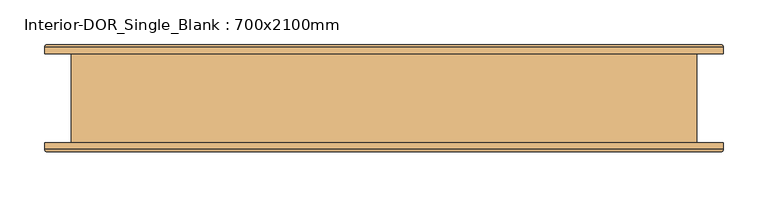
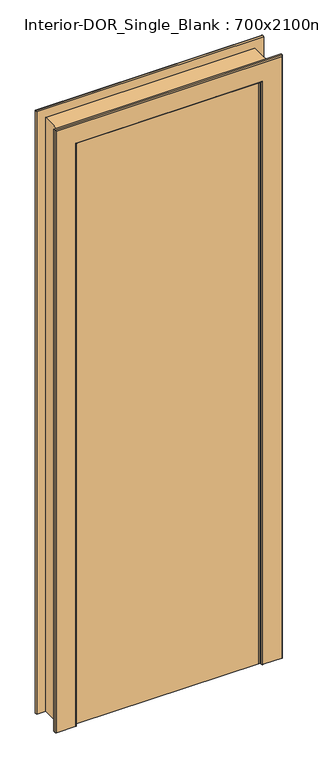
"""IFC4 building model written with IfcOpenShell, lengths in millimetres: door geometry, Interior-DOR_Single_Blank : 700x2100mm."""

import ifcopenshell
import ifcopenshell.guid

model = None  # the IFC model being written
_history = None  # IfcOwnerHistory: only IFC2X3 demands one
_inside = {}  # id of a spatial element -> (the spatial element, [elements in it])
_under = {}  # id of a project, library or spatial element -> (it, [spatial elements below it])
_declared = {}  # id of a project -> (the project, [libraries it declares])
_typed = {}  # id of a type object -> (the type object, [elements of that type])
_made_of = {}  # id of a material, layer set ... -> (it, [elements and type objects made of it])


def new_model(schema):
    """Start an empty IFC model of exactly this schema.

    Asked for "IFC4X3", IfcOpenShell would pick the latest addendum, in which some entities
    have other attributes; the version numbers below select the first issue.
    IFC2X3 requires an IfcOwnerHistory on every rooted entity: one is made here for all.
    """
    global model, _history
    if schema == "IFC4X3":
        model = ifcopenshell.file(schema_version=(4, 3, 0, 0))
    else:
        model = ifcopenshell.file(schema=schema)
    _inside.clear()
    _under.clear()
    _declared.clear()
    _typed.clear()
    _made_of.clear()
    _history = None
    if model.schema == "IFC2X3":
        org = make("IfcOrganization", Name="unknown")
        user = make(
            "IfcPersonAndOrganization",
            ThePerson=make("IfcPerson", FamilyName="unknown"),
            TheOrganization=org,
        )
        app = make(
            "IfcApplication",
            ApplicationDeveloper=org,
            Version="unknown",
            ApplicationFullName="unknown",
            ApplicationIdentifier="unknown",
        )
        _history = make(
            "IfcOwnerHistory",
            OwningUser=user,
            OwningApplication=app,
            ChangeAction="ADDED",
            CreationDate=0,
        )
    return model


def make(cls, **values):
    """One entity of the class cls with the attributes given. An attribute that is None is left unset."""
    return model.create_entity(
        cls, **{name: value for name, value in values.items() if value is not None}
    )


def rooted(cls, **values):
    """An entity with a GlobalId (a new one), such as an element, a storey or a relation."""
    return make(cls, GlobalId=ifcopenshell.guid.new(), OwnerHistory=_history, **values)


def si_unit(unit_type, name, prefix=None):
    """IfcSIUnit, for example si_unit("LENGTHUNIT", "METRE", prefix="MILLI")."""
    return make("IfcSIUnit", UnitType=unit_type, Prefix=prefix, Name=name)


def assignment(units):
    """IfcUnitAssignment: the units of a project."""
    return None if units is None else make("IfcUnitAssignment", Units=units)


def point(xyz):
    """IfcCartesianPoint."""
    return None if xyz is None else make("IfcCartesianPoint", Coordinates=xyz)


def direction(xyz):
    """IfcDirection."""
    return None if xyz is None else make("IfcDirection", DirectionRatios=xyz)


def frame(location, z_axis=None, x_axis=None):
    """IfcAxis2Placement3D, a coordinate frame: its origin and axes. An axis left out is left unset."""
    return make(
        "IfcAxis2Placement3D",
        Location=point(location),
        Axis=direction(z_axis),
        RefDirection=direction(x_axis),
    )


def origin():
    """The frame at (0, 0, 0) with its axes left unset."""
    return frame((0.0, 0.0, 0.0))


def origin_with_axes():
    """The frame at (0, 0, 0) with the z axis (0, 0, 1) and the x axis (1, 0, 0) written out."""
    return frame((0.0, 0.0, 0.0), z_axis=(0.0, 0.0, 1.0), x_axis=(1.0, 0.0, 0.0))


def place(relative_to, where):
    """IfcLocalPlacement: puts the frame where relative to a parent placement (None: the world)."""
    return make(
        "IfcLocalPlacement", PlacementRelTo=relative_to, RelativePlacement=where
    )


def context(
    kind, dimensions, precision=None, world=None, true_north=None, identifier=None
):
    """IfcGeometricRepresentationContext, for example the 3D "Model" context."""
    return make(
        "IfcGeometricRepresentationContext",
        ContextIdentifier=identifier,
        ContextType=kind,
        CoordinateSpaceDimension=dimensions,
        Precision=precision,
        WorldCoordinateSystem=world,
        TrueNorth=true_north,
    )


def project(units=None, contexts=None):
    """IfcProject with its units and contexts."""
    return rooted(
        "IfcProject",
        Name="project",
        RepresentationContexts=contexts,
        UnitsInContext=assignment(units),
    )


def spatial(cls, under=None, at=None, **own):
    """A site, building, storey or space (cls), placed at a placement, below another one or the project."""
    s = rooted(cls, ObjectPlacement=at, **own)
    if under is not None:
        _under.setdefault(under.id(), (under, []))[1].append(s)
    return s


def polyline(points):
    """IfcPolyline through the points."""
    return make("IfcPolyline", Points=[point(p) for p in points])


def circle_curve(where, radius):
    """IfcCircle in the frame where."""
    return make("IfcCircle", Position=where, Radius=radius)


def ellipse_curve(where, semi_axis1, semi_axis2):
    """IfcEllipse in the frame where."""
    return make(
        "IfcEllipse", Position=where, SemiAxis1=semi_axis1, SemiAxis2=semi_axis2
    )


def outline(outer, holes=None, kind="AREA"):
    """IfcArbitraryClosedProfileDef: a profile drawn as a closed curve; with holes, ...WithVoids."""
    if holes is None:
        return make("IfcArbitraryClosedProfileDef", ProfileType=kind, OuterCurve=outer)
    return make(
        "IfcArbitraryProfileDefWithVoids",
        ProfileType=kind,
        OuterCurve=outer,
        InnerCurves=holes,
    )


def extrude(swept, where, along, depth):
    """IfcExtrudedAreaSolid: the profile swept, set in the frame where, extruded along a direction by depth."""
    return make(
        "IfcExtrudedAreaSolid",
        SweptArea=swept,
        Position=where,
        ExtrudedDirection=direction(along),
        Depth=depth,
    )


def faces_of(points, faces, orient=None, outer=None):
    """IfcFace entities. A face is a list of loops; a loop is a list of indices into points, from 0.

    orient and outer hold one flag for each loop. By default every Orientation is true, the
    first loop of a face is its IfcFaceOuterBound and the others are IfcFaceBound.
    """
    made = []
    for i, loops in enumerate(faces):
        bounds = []
        for j, loop in enumerate(loops):
            is_outer = j == 0 if outer is None else outer[i][j]
            bounds.append(
                make(
                    "IfcFaceOuterBound" if is_outer else "IfcFaceBound",
                    Bound=make("IfcPolyLoop", Polygon=[points[k] for k in loop]),
                    Orientation=True if orient is None else orient[i][j],
                )
            )
        made.append(make("IfcFace", Bounds=bounds))
    return made


def faceted_brep(points, faces, orient=None, outer=None, voids=None):
    """IfcFacetedBrep: a solid bounded by flat faces; with voids (closed shells), ...WithVoids."""
    shared = [point(p) for p in points]
    hull = make("IfcClosedShell", CfsFaces=faces_of(shared, faces, orient, outer))
    if voids is None:
        return make("IfcFacetedBrep", Outer=hull)
    return make(
        "IfcFacetedBrepWithVoids",
        Outer=hull,
        Voids=[
            make(cls, CfsFaces=faces_of(shared, fs, o, b)) for cls, fs, o, b in voids
        ],
    )


def shape(context_of_items, identifier, shape_type, items):
    """IfcShapeRepresentation: the items that make up one representation, for example the "Body"."""
    return make(
        "IfcShapeRepresentation",
        ContextOfItems=context_of_items,
        RepresentationIdentifier=identifier,
        RepresentationType=shape_type,
        Items=items,
    )


def source(mapping_origin, context_of_items, identifier, shape_type, items):
    """IfcRepresentationMap: a shape defined once, which mapped items show again and again."""
    return make(
        "IfcRepresentationMap",
        MappingOrigin=mapping_origin,
        MappedRepresentation=shape(context_of_items, identifier, shape_type, items),
    )


def transform(
    local_origin,
    x_axis=None,
    y_axis=None,
    z_axis=None,
    scale=None,
    scale2=None,
    scale3=None,
    uniform=True,
):
    """IfcCartesianTransformationOperator3D, or its non-uniform kind. x_axis, y_axis, z_axis: its Axis1, 2, 3."""
    if uniform:
        return make(
            "IfcCartesianTransformationOperator3D",
            Axis1=direction(x_axis),
            Axis2=direction(y_axis),
            LocalOrigin=point(local_origin),
            Scale=scale,
            Axis3=direction(z_axis),
        )
    return make(
        "IfcCartesianTransformationOperator3DnonUniform",
        Axis1=direction(x_axis),
        Axis2=direction(y_axis),
        LocalOrigin=point(local_origin),
        Scale=scale,
        Axis3=direction(z_axis),
        Scale2=scale2,
        Scale3=scale3,
    )


def mapped(mapping_source, mapping_target):
    """IfcMappedItem: shows the shape of a source again, moved by a transform."""
    return make(
        "IfcMappedItem", MappingSource=mapping_source, MappingTarget=mapping_target
    )


def made_of(thing, what):
    """Note that an element or type object is made of a material, layer set ...; save() writes the relation."""
    if what is not None:
        _made_of.setdefault(what.id(), (what, []))[1].append(thing)
    return thing


def element(
    cls,
    number,
    at=None,
    inside=None,
    cuts=None,
    type_object=None,
    material=None,
    context=None,
    identifier="Body",
    shape_type=None,
    held_by="IfcProductDefinitionShape",
    body=None,
    shapes=None,
    **own,
):
    """One element of the class cls, such as IfcWall. Its Tag is "e" and its number.

    at: its placement. inside: the storey or other place that contains it. cuts: it is an
    opening in that element (IfcRelVoidsElement). A single representation is given by context,
    identifier, shape_type and body (its items); several are given by shapes. held_by: the class
    of the entity that holds the representations. save() writes the other relations.
    """
    e = rooted(cls, Tag="e%d" % number, ObjectPlacement=at, **own)
    if body is not None:
        shapes = [shape(context, identifier, shape_type, body)]
    if shapes is not None:
        e.Representation = make(held_by, Representations=shapes)
    if inside is not None:
        _inside.setdefault(inside.id(), (inside, []))[1].append(e)
    if cuts is not None:
        rooted(
            "IfcRelVoidsElement", RelatingBuildingElement=cuts, RelatedOpeningElement=e
        )
    if type_object is not None:
        _typed.setdefault(type_object.id(), (type_object, []))[1].append(e)
    return made_of(e, material)


def aggregate(whole, parts):
    """IfcRelAggregates: a whole, such as a stair, and the parts it consists of."""
    return rooted("IfcRelAggregates", RelatingObject=whole, RelatedObjects=parts)


def save(model, path):
    """Write the relations noted so far, then the file.

    IfcRelAggregates (storeys below a building ...), IfcRelContainedInSpatialStructure (elements
    in a storey), IfcRelDefinesByType, IfcRelAssociatesMaterial and IfcRelDeclares: one each for
    every whole, place, type object, material and project.
    """
    for whole, parts in _under.values():
        aggregate(whole, parts)
    for where, things in _inside.values():
        rooted(
            "IfcRelContainedInSpatialStructure",
            RelatedElements=things,
            RelatingStructure=where,
        )
    for kind, things in _typed.values():
        rooted("IfcRelDefinesByType", RelatedObjects=things, RelatingType=kind)
    for what, things in _made_of.values():
        rooted("IfcRelAssociatesMaterial", RelatedObjects=things, RelatingMaterial=what)
    for by, libraries in _declared.values():
        rooted("IfcRelDeclares", RelatingContext=by, RelatedDefinitions=libraries)
    model.write(path)


def plane_surface(at):
    """IfcPlane: the flat surface through the origin of the frame at, square to its z axis."""
    return make("IfcPlane", Position=at)


def cylinder_surface(at, radius):
    """IfcCylindricalSurface: all points at the distance radius from the z axis of the frame at."""
    return make("IfcCylindricalSurface", Position=at, Radius=radius)


def advanced_brep(points, edges, surfaces, faces):
    """IfcAdvancedBrep: a solid bounded by faces that lie on surfaces and meet in shared edges.

    An edge is (start, end): straight between two places in points (the first is 0);
    or (start, end, curve); or (start, end, curve, False) where it runs against its curve.
    A face is (place in surfaces, loops), or (place, loops, False) where it looks against
    its surface's normal. A loop lists edges by number (the first is 1), with a minus sign
    where the edge is run from its end to its start. The first loop is the outer one.
    """
    corners = [point(p) for p in points]
    vertices = [make("IfcVertexPoint", VertexGeometry=c) for c in corners]
    made = []
    for start, end, *more in edges:
        made.append(
            make(
                "IfcEdgeCurve",
                EdgeStart=vertices[start],
                EdgeEnd=vertices[end],
                EdgeGeometry=more[0] if more else make("IfcPolyline", Points=[corners[start], corners[end]]),
                SameSense=more[1] if len(more) > 1 else True,
            )
        )
    hull = []
    for where, loops, *sense in faces:
        bounds = []
        for j, loop in enumerate(loops):
            ring = [make("IfcOrientedEdge", EdgeElement=made[abs(k) - 1], Orientation=k > 0) for k in loop]
            bounds.append(
                make(
                    "IfcFaceOuterBound" if j == 0 else "IfcFaceBound",
                    Bound=make("IfcEdgeLoop", EdgeList=ring),
                    Orientation=True,
                )
            )
        hull.append(make("IfcAdvancedFace", Bounds=bounds, FaceSurface=surfaces[where], SameSense=sense[0] if sense else True))
    return make("IfcAdvancedBrep", Outer=make("IfcClosedShell", CfsFaces=hull))


def interior_dor_single_blank_700x2100mm_7bd7bfec(model_context):
    return source(origin(), model_context, "Body", "SolidModel", [
        advanced_brep(
        [(-310.0, -50.0, 0.0), (-310.0, -57.0, 0.0), (-313.0, -60.0, 0.0), (-377.0, -60.0, 0.0), (-380.0, -57.0, 0.0), (-380.0, -50.0, 0.0), (-310.0, -50.0, 2060.0), (-310.0, -57.0, 2060.0), (-313.0, -60.0, 2063.0), (313.0, -60.0, 2063.0), (313.0, -60.0, 0.0), (377.0, -60.0, 0.0), (377.0, -60.0, 2127.0), (-377.0, -60.0, 2127.0), (-380.0, -57.0, 2130.0), (-380.0, -50.0, 2130.0), (380.0, -50.0, 2130.0), (380.0, -50.0, 0.0), (310.0, -50.0, 0.0), (310.0, -50.0, 2060.0), (310.0, -57.0, 2060.0), (310.0, -57.0, 0.0), (380.0, -57.0, 0.0), (380.0, -57.0, 2130.0)],
        [
            (0, 1),
            (1, 2, circle_curve(frame((-313.0, -57.0, 0.0), z_axis=(0.0, 0.0, -1.0), x_axis=(-1.0, 0.0, 0.0)), 3.0)),
            (2, 3),
            (3, 4, circle_curve(frame((-377.0, -57.0, 0.0), z_axis=(0.0, 0.0, -1.0), x_axis=(-1.0, 0.0, 0.0)), 3.0)),
            (4, 5),
            (5, 0),
            (0, 6),
            (6, 7),
            (7, 1),
            (7, 8, ellipse_curve(frame((-313.0, -57.0, 2063.0), z_axis=(-0.7071067811865475, 0.0, -0.7071067811865475), x_axis=(0.7071067811865474, 0.0, -0.7071067811865476)), 4.2426407, 3.0)),
            (8, 2),
            (8, 9),
            (9, 10),
            (10, 11),
            (11, 12),
            (12, 13),
            (13, 3),
            (13, 14, ellipse_curve(frame((-377.0, -57.0, 2127.0), z_axis=(-0.7071067811865475, 0.0, -0.7071067811865475), x_axis=(0.7071067811865474, 0.0, -0.7071067811865476)), 4.2426407, 3.0)),
            (14, 4),
            (14, 15),
            (15, 5),
            (15, 16),
            (16, 17),
            (17, 18),
            (18, 19),
            (19, 6),
            (9, 20, ellipse_curve(frame((313.0, -57.0, 2063.0), z_axis=(0.7071067811865475, 0.0, -0.7071067811865475), x_axis=(0.7071067811865474, 0.0, 0.7071067811865476)), 4.2426407, 3.0)),
            (20, 21),
            (21, 10, circle_curve(frame((313.0, -57.0, 0.0), z_axis=(0.0, 0.0, 1.0), x_axis=(1.0, 0.0, 0.0)), 3.0)),
            (17, 22),
            (22, 11, circle_curve(frame((377.0, -57.0, 0.0), z_axis=(0.0, 0.0, -1.0), x_axis=(1.0, 0.0, 0.0)), 3.0)),
            (21, 18),
            (23, 12, ellipse_curve(frame((377.0, -57.0, 2127.0), z_axis=(0.7071067811865475, 0.0, -0.7071067811865475), x_axis=(0.7071067811865474, 0.0, 0.7071067811865476)), 4.2426407, 3.0)),
            (22, 23),
            (16, 23),
            (20, 19),
            (20, 7),
            (23, 14),
        ],
        [
            plane_surface(frame((-350.0, 50.0, 0.0), z_axis=(0.0, 0.0, -1.0), x_axis=(0.0, -1.0, 0.0))),
            plane_surface(frame((-310.0, -50.0, 0.0), z_axis=(1.0, 0.0, 0.0), x_axis=(0.0, 0.0, 1.0))),
            cylinder_surface(frame((-313.0, -57.0, 0.0), z_axis=(0.0, 0.0, -1.0), x_axis=(-1.0, 0.0, 0.0)), 3.0),
            plane_surface(frame((-313.0, -60.0, 0.0), z_axis=(0.0, -1.0, 0.0), x_axis=(0.0, 0.0, 1.0))),
            cylinder_surface(frame((-377.0, -57.0, 0.0), z_axis=(0.0, 0.0, -1.0), x_axis=(-1.0, 0.0, 0.0)), 3.0),
            plane_surface(frame((-380.0, -57.0, 0.0), z_axis=(-1.0, 0.0, 0.0), x_axis=(0.0, 0.0, 1.0))),
            plane_surface(frame((-380.0, -50.0, 0.0), z_axis=(0.0, 1.0, 0.0), x_axis=(0.0, 0.0, 1.0))),
            cylinder_surface(frame((313.0, -57.0, 2100.0), z_axis=(0.0, 0.0, 1.0), x_axis=(1.0, 0.0, 0.0)), 3.0),
            plane_surface(frame((350.0, 50.0, 0.0), z_axis=(0.0, 0.0, -1.0), x_axis=(0.0, -1.0, 0.0))),
            cylinder_surface(frame((377.0, -57.0, 2100.0), z_axis=(0.0, 0.0, 1.0), x_axis=(1.0, 0.0, 0.0)), 3.0),
            plane_surface(frame((380.0, -57.0, 2130.0), z_axis=(1.0, 0.0, 0.0), x_axis=(0.0, 0.0, -1.0))),
            plane_surface(frame((310.0, -50.0, 2060.0), z_axis=(-1.0, 0.0, 0.0), x_axis=(0.0, 0.0, -1.0))),
            plane_surface(frame((-310.0, -50.0, 2060.0), z_axis=(0.0, 0.0, -1.0), x_axis=(1.0, 0.0, 0.0))),
            cylinder_surface(frame((-350.0, -57.0, 2063.0), z_axis=(-1.0, 0.0, 0.0), x_axis=(0.0, 0.0, 1.0)), 3.0),
            cylinder_surface(frame((-350.0, -57.0, 2127.0), z_axis=(-1.0, 0.0, 0.0), x_axis=(0.0, 0.0, 1.0)), 3.0),
            plane_surface(frame((-380.0, -57.0, 2130.0), z_axis=(0.0, 0.0, 1.0), x_axis=(1.0, 0.0, 0.0))),
        ],
        [
            (0, [[1, 2, 3, 4, 5, 6]]),
            (1, [[-1, 7, 8, 9]]),
            (2, [[-2, -9, 10, 11]]),
            (3, [[-3, -11, 12, 13, 14, 15, 16, 17]]),
            (4, [[-4, -17, 18, 19]]),
            (5, [[-5, -19, 20, 21]]),
            (6, [[-6, -21, 22, 23, 24, 25, 26, -7]]),
            (7, [[27, 28, 29, -13]]),
            (8, [[-24, 30, 31, -14, -29, 32]]),
            (9, [[33, -15, -31, 34]]),
            (10, [[35, -34, -30, -23]]),
            (11, [[36, -25, -32, -28]]),
            (12, [[-8, -26, -36, 37]]),
            (13, [[-10, -37, -27, -12]]),
            (14, [[-18, -16, -33, 38]]),
            (15, [[-20, -38, -35, -22]]),
        ],
    ),
        advanced_brep(
        [(-380.0, 50.0, 0.0), (-380.0, 57.0, 0.0), (-377.0, 60.0, 0.0), (-313.0, 60.0, 0.0), (-310.0, 57.0, 0.0), (-310.0, 50.0, 0.0), (-380.0, 50.0, 2130.0), (-380.0, 57.0, 2130.0), (-377.0, 60.0, 2127.0), (377.0, 60.0, 2127.0), (377.0, 60.0, 0.0), (313.0, 60.0, 0.0), (313.0, 60.0, 2063.0), (-313.0, 60.0, 2063.0), (-310.0, 57.0, 2060.0), (-310.0, 50.0, 2060.0), (310.0, 50.0, 2060.0), (310.0, 50.0, 0.0), (380.0, 50.0, 0.0), (380.0, 50.0, 2130.0), (380.0, 57.0, 2130.0), (380.0, 57.0, 0.0), (310.0, 57.0, 0.0), (310.0, 57.0, 2060.0)],
        [
            (0, 1),
            (1, 2, circle_curve(frame((-377.0, 57.0, 0.0), z_axis=(0.0, 0.0, -1.0), x_axis=(-1.0, 0.0, 0.0)), 3.0)),
            (2, 3),
            (3, 4, circle_curve(frame((-313.0, 57.0, 0.0), z_axis=(0.0, 0.0, -1.0), x_axis=(-1.0, 0.0, 0.0)), 3.0)),
            (4, 5),
            (5, 0),
            (0, 6),
            (6, 7),
            (7, 1),
            (7, 8, ellipse_curve(frame((-377.0, 57.0, 2127.0), z_axis=(-0.7071067811865475, 0.0, -0.7071067811865475), x_axis=(0.7071067811865474, 0.0, -0.7071067811865476)), 4.2426407, 3.0)),
            (8, 2),
            (8, 9),
            (9, 10),
            (10, 11),
            (11, 12),
            (12, 13),
            (13, 3),
            (13, 14, ellipse_curve(frame((-313.0, 57.0, 2063.0), z_axis=(-0.7071067811865475, 0.0, -0.7071067811865475), x_axis=(0.7071067811865474, 0.0, -0.7071067811865476)), 4.2426407, 3.0)),
            (14, 4),
            (14, 15),
            (15, 5),
            (15, 16),
            (16, 17),
            (17, 18),
            (18, 19),
            (19, 6),
            (9, 20, ellipse_curve(frame((377.0, 57.0, 2127.0), z_axis=(0.7071067811865475, 0.0, -0.7071067811865475), x_axis=(0.7071067811865474, 0.0, 0.7071067811865476)), 4.2426407, 3.0)),
            (20, 21),
            (21, 10, circle_curve(frame((377.0, 57.0, 0.0), z_axis=(0.0, 0.0, 1.0), x_axis=(1.0, 0.0, 0.0)), 3.0)),
            (17, 22),
            (22, 11, circle_curve(frame((313.0, 57.0, 0.0), z_axis=(0.0, 0.0, -1.0), x_axis=(1.0, 0.0, 0.0)), 3.0)),
            (21, 18),
            (23, 12, ellipse_curve(frame((313.0, 57.0, 2063.0), z_axis=(0.7071067811865475, 0.0, -0.7071067811865475), x_axis=(0.7071067811865474, 0.0, 0.7071067811865476)), 4.2426407, 3.0)),
            (22, 23),
            (16, 23),
            (20, 19),
            (20, 7),
            (23, 14),
        ],
        [
            plane_surface(frame((-350.0, 50.0, 0.0), z_axis=(0.0, 0.0, -1.0), x_axis=(0.0, -1.0, 0.0))),
            plane_surface(frame((-380.0, 50.0, 0.0), z_axis=(-1.0, 0.0, 0.0), x_axis=(0.0, 0.0, 1.0))),
            cylinder_surface(frame((-377.0, 57.0, 0.0), z_axis=(0.0, 0.0, -1.0), x_axis=(-1.0, 0.0, 0.0)), 3.0),
            plane_surface(frame((-377.0, 60.0, 0.0), z_axis=(0.0, 1.0, 0.0), x_axis=(0.0, 0.0, 1.0))),
            cylinder_surface(frame((-313.0, 57.0, 0.0), z_axis=(0.0, 0.0, -1.0), x_axis=(-1.0, 0.0, 0.0)), 3.0),
            plane_surface(frame((-310.0, 57.0, 0.0), z_axis=(1.0, 0.0, 0.0), x_axis=(0.0, 0.0, 1.0))),
            plane_surface(frame((-310.0, 50.0, 0.0), z_axis=(0.0, -1.0, 0.0), x_axis=(0.0, 0.0, 1.0))),
            cylinder_surface(frame((377.0, 57.0, 2100.0), z_axis=(0.0, 0.0, 1.0), x_axis=(1.0, 0.0, 0.0)), 3.0),
            plane_surface(frame((350.0, 50.0, 0.0), z_axis=(0.0, 0.0, -1.0), x_axis=(0.0, -1.0, 0.0))),
            cylinder_surface(frame((313.0, 57.0, 2100.0), z_axis=(0.0, 0.0, 1.0), x_axis=(1.0, 0.0, 0.0)), 3.0),
            plane_surface(frame((310.0, 57.0, 2060.0), z_axis=(-1.0, 0.0, 0.0), x_axis=(0.0, 0.0, -1.0))),
            plane_surface(frame((380.0, 50.0, 2130.0), z_axis=(1.0, 0.0, 0.0), x_axis=(0.0, 0.0, -1.0))),
            plane_surface(frame((-380.0, 50.0, 2130.0), z_axis=(0.0, 0.0, 1.0), x_axis=(1.0, 0.0, 0.0))),
            cylinder_surface(frame((-350.0, 57.0, 2127.0), z_axis=(-1.0, 0.0, 0.0), x_axis=(0.0, 0.0, 1.0)), 3.0),
            cylinder_surface(frame((-350.0, 57.0, 2063.0), z_axis=(-1.0, 0.0, 0.0), x_axis=(0.0, 0.0, 1.0)), 3.0),
            plane_surface(frame((-310.0, 57.0, 2060.0), z_axis=(0.0, 0.0, -1.0), x_axis=(1.0, 0.0, 0.0))),
        ],
        [
            (0, [[1, 2, 3, 4, 5, 6]]),
            (1, [[-1, 7, 8, 9]]),
            (2, [[-2, -9, 10, 11]]),
            (3, [[-3, -11, 12, 13, 14, 15, 16, 17]]),
            (4, [[-4, -17, 18, 19]]),
            (5, [[-5, -19, 20, 21]]),
            (6, [[-6, -21, 22, 23, 24, 25, 26, -7]]),
            (7, [[27, 28, 29, -13]]),
            (8, [[-24, 30, 31, -14, -29, 32]]),
            (9, [[33, -15, -31, 34]]),
            (10, [[35, -34, -30, -23]]),
            (11, [[36, -25, -32, -28]]),
            (12, [[-8, -26, -36, 37]]),
            (13, [[-10, -37, -27, -12]]),
            (14, [[-18, -16, -33, 38]]),
            (15, [[-20, -38, -35, -22]]),
        ],
    ),
        faceted_brep([(-350.0, 50.0, 0.0), (-305.0, 50.0, 0.0), (-305.0, 35.0, 0.0), (-285.0, 35.0, 0.0), (-285.0, -5.0, 0.0), (-305.0, -5.0, 0.0), (-305.0, -50.0, 0.0), (-350.0, -50.0, 0.0), (-350.0, 50.0, 2100.0), (350.0, 50.0, 2100.0), (350.0, 50.0, 0.0), (305.0, 50.0, 0.0), (305.0, 50.0, 2055.0), (-305.0, 50.0, 2055.0), (-305.0, 35.0, 2055.0), (305.0, 35.0, 2055.0), (305.0, 35.0, 0.0), (285.0, 35.0, 0.0), (285.0, 35.0, 2035.0), (-285.0, 35.0, 2035.0), (-285.0, -5.0, 2035.0), (285.0, -5.0, 2035.0), (285.0, -5.0, 0.0), (305.0, -5.0, 0.0), (305.0, -5.0, 2055.0), (-305.0, -5.0, 2055.0), (-305.0, -50.0, 2055.0), (305.0, -50.0, 2055.0), (305.0, -50.0, 0.0), (350.0, -50.0, 0.0), (350.0, -50.0, 2100.0), (-350.0, -50.0, 2100.0)], [[[0, 1, 2, 3, 4, 5, 6, 7]], [[1, 0, 8, 9, 10, 11, 12, 13]], [[2, 1, 13, 14]], [[3, 2, 14, 15, 16, 17, 18, 19]], [[4, 3, 19, 20]], [[5, 4, 20, 21, 22, 23, 24, 25]], [[6, 5, 25, 26]], [[7, 6, 26, 27, 28, 29, 30, 31]], [[0, 7, 31, 8]], [[9, 30, 29, 10]], [[10, 29, 28, 23, 22, 17, 16, 11]], [[15, 12, 11, 16]], [[21, 18, 17, 22]], [[27, 24, 23, 28]], [[20, 19, 18, 21]], [[26, 25, 24, 27]], [[8, 31, 30, 9]], [[14, 13, 12, 15]]]),
        extrude(outline(polyline([(305.0, -50.0), (-305.0, -50.0), (-305.0, -5.0), (305.0, -5.0), (305.0, -50.0)])), origin_with_axes(), (0.0, 0.0, 1.0), 2055.0),
    ])


if __name__ == "__main__":
    model = new_model("IFC4")
    model_context = context("Model", 3, world=origin())
    ifc_project = project(units=[si_unit("LENGTHUNIT", "METRE", prefix="MILLI")], contexts=[model_context])
    site = spatial("IfcSite", under=ifc_project)
    building = spatial("IfcBuilding", under=site)
    placement = place(None, origin())
    interior_dor_single_blank_700x2100mm_shape = interior_dor_single_blank_700x2100mm_7bd7bfec(model_context)
    element("IfcDoor", 1, ObjectType="Interior-DOR_Single_Blank : 700x2100mm", at=placement, inside=building, context=model_context, shape_type="MappedRepresentation", body=[
        mapped(interior_dor_single_blank_700x2100mm_shape, transform((0.0, 0.0, 0.0), x_axis=(1.0, 0.0, 0.0), y_axis=(0.0, 1.0, 0.0), z_axis=(0.0, 0.0, 1.0))),
    ])
    save(model, "model.ifc")

# Revit data of these elements
# Type "Interior-DOR_Single_Blank : 700x2100mm"
#   Type IfcGUID = "1sWU2cMPP4xwRoAc3TXQKN"
#   Assembly Code = "C1020120"
#   Type Mark = "196"
#   Classification.Uniclass.EF.Number = "EF_25_30"
#   Classification.Uniclass.EF.Description = "Doors and windows"
#   WindLoadRating = "n/a"
#   WaterTightnessRating = "n/a"
#   WarrantyStartDate [instance default] = "1900-12-31T23:59:59"
#   WarrantyGuarantorParts = "n/a"
#   WarrantyGuarantorLabor = "n/a"
#   WarrantyDurationUnit = "year"
#   WarrantyDurationParts = "n/a"
#   WarrantyDurationLabor = "n/a"
#   WarrantyDescription = "n/a"
#   Version = "2"
#   Uniclass2015Version = "Systems v1.9"
#   Uniclass2015Title = "Doorset systems"
#   Uniclass2015Code = "Ss_25_30_20_25"
#   URL = "www.nationalbimlibrary.com"
#   TagNumber [instance default] = "n/a"
#   SustainabilityPerformance = "n/a"
#   Status = "UNSET"
#   Size = "1010 x 2100 mm"
#   Shape = "n/a"
#   SerialNumber [instance default] = "n/a"
#   SecurityRating = "n/a"
#   Revision = "n/a"
#   ReplacementCost = "n/a"
#   Reference = "n/a"
#   ProductInformation = "n/a"
#   Operation = "SINGLE_SWING_RIGHT"
#   OmniClassVersion = "Table 22 2012-05-16"
#   OmniClassTitle = "Doors and Frames"
#   OmniClassCode = "22-08 10 00"
#   Name = "DoorsetSystem_Interior-Single_Blank"
#   NBSReference = "25-50-20/120"
#   NBSDescription = "Doorset system"
#   NBSCertification = "www.nationalbimlibrary.com/cert/mlf45nxc"
#   ModelReference = "Interior Single Door"
#   ModelNumber = "n/a"
#   Model = "Interior Single Door"
#   MechanicalLoadRating = "n/a"
#   Material = "n/a"
#   ManufacturerURL = "n/a"
#   ManufacturerName = "n/a"
#   Manufacturer = "info@theNBS.com"
#   InstallationDate [instance default] = "1900-12-31T23:59:59"
#   IfcExportType = "DOOR"
#   IfcExportAs = "IfcDoorType"
#   HygrothermalRating = "n/a"
#   Grade = "n/a"
#   FireRating = "n/a"
#   Fire Rating = "n/a"
#   Finish = "n/a"
#   Features = "n/a"
#   ExpectedLife = "n/a"
#   DurationUnit = "n/a"
#   DurabilityRating = "n/a"
#   DoorNumber [instance default] = "n/a"
#   Description = "Generic single interior door"
#   Construction Type = "USERDEFINED"
#   Constituents = "n/a"
#   ComponentNumber [instance default] = "n/a"
#   Color = "n/a"
#   CodePerformance = "n/a"
#   Category = "Ss_25_30_20_25:Doorset systems"
#   BarCode [instance default] = "n/a"
#   BIMObjectName = "NBS_DoorsetSystem_Interior-Single_Blank"
#   Author = "NBS"
#   AssetType = "Fixed"
#   AssetIdentifier [instance default] = "n/a"
#   AcousticRating = "n/a"
#   AccessibilityPerformance = "n/a"
#   Width = 0.7 m
#   WallThickness [instance default] = 0.15 m
#   ThresholdHeight = 0.015 m
#   Thickness = 0.15 m
#   ThermalTransmittance = 0
#   StructuralToleranceJamb = 0 m
#   StructuralToleranceHead = 0 m
#   StructuralOpeningWidth = 0.7 m
#   StructuralOpeningHeight = 2.1 m
#   StopProjection = 0.02 m
#   StopDepth = 0.04 m
#   Rough Width [instance default] = 0.7 m
#   Rough Height [instance default] = 2.1 m
#   RebateDepth = 0.045 m
#   PanelWidth = 0.61 m
#   PanelUndercut = 0 m
#   PanelHeight = 2.055 m
#   PanelDepth = 0.045 m
#   OpeningTolerance = 0 m
#   NominalWidth = 0.7 m
#   NominalLength = 0 m
#   NominalHeight = 2.1 m
#   Infiltration = 0
#   Height = 2.1 m
#   GlazingAreaFraction = 0
#   FrameThickness = 0.045 m
#   FrameSetback [instance default] = 0 m
#   FrameDepth [instance default] = 0.15 m
#   FinishThicknessInternal [instance default] = 0 m
#   FinishThicknessExternal [instance default] = 0 m
#   ClearOpeningWidth = 0.57 m
#   ClearOpeningHeight = 2.035 m
#   CalculatedInteriorVoidDepth [instance default] = 0.3 m
#   ArchitraveWidth = 0.07 m
#   ArchitraveThickness = 0.01 m
#   ArchitraveSetbackFromFrameFace = 0.005 m
#   SmokeStop = no
#   SingleRebate = no
#   SelfClosing = no
#   PlantedStop = yes
#   IsExternal = no
#   HasDrive = no
#   HandicapAccessible = no
#   Wall Closure = 4
#   FireExit = no
#   ArchitraveFrontRequired [instance default] = yes
#   ArchitraveBackRequired [instance default] = yes
#   PanelMaterial = NBS_Concept
#   HardwareFinish = NBS_Concept
#   FrameSectionMaterial = NBS_Concept
#   Function = (empty or 0)
#   Cost = 0
# Element 1 (IfcDoor, "Interior-DOR_Single_Blank : 700x2100mm")
#   WallThickness = 0.1 m
#   FrameDepth = 0.1 m
#   Materials on its faces: "NBS_Concept"
# Materials
#   "NBS_Concept": class "Generic", colour RGB 255 255 255, transparency 0, Description = "To be specified", Cost = 0
